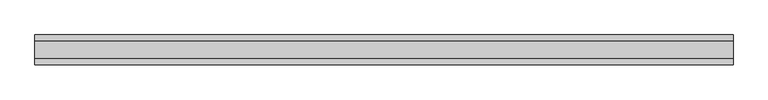
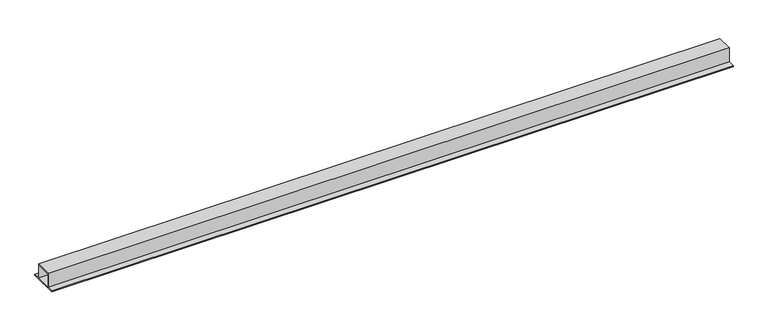
"""IFC4 building model written with IfcOpenShell, lengths in millimetres: beam geometry, NLRS_28_SF_LIB_stalen ligger THQ-AV-CWV-MMBS-SRP_gen_rsf : stalen ligger_gen__THQ_280x10-290x30-550x20."""

from ifc_helpers import new_model, si_unit, frame, origin, place, context, project, spatial, polyline, outline, extrude, source, transform, mapped, element, save


def beam_736acf17(model_context):
    return source(origin(), model_context, "Body", "SweptSolid", [
        extrude(outline(polyline([(143.5, 280.0), (143.5, 0.0), (263.5, 0.0), (263.5, -20.0), (-286.5, -20.0), (-286.5, 0.0), (-166.5, 0.0), (-166.5, 280.0), (143.5, 280.0)]), holes=[polyline([(133.5, 0.0), (133.5, 250.0), (-156.5, 250.0), (-156.5, 0.0), (133.5, 0.0)])]), frame((-6445.0, 0.0, 0.0), z_axis=(1.0, 0.0, 0.0), x_axis=(0.0, 1.0, 0.0)), (0.0, 0.0, 1.0), 12890.0),
    ])


if __name__ == "__main__":
    model = new_model("IFC4")
    model_context = context("Model", 3, world=origin())
    ifc_project = project(units=[si_unit("LENGTHUNIT", "METRE", prefix="MILLI")], contexts=[model_context])
    site = spatial("IfcSite", under=ifc_project)
    building = spatial("IfcBuilding", under=site)
    placement = place(None, origin())
    beam_shape = beam_736acf17(model_context)
    element("IfcBeam", 1, ObjectType="NLRS_28_SF_LIB_stalen ligger THQ-AV-CWV-MMBS-SRP_gen_rsf : stalen ligger_gen__THQ_280x10-290x30-550x20", at=placement, inside=building, context=model_context, shape_type="MappedRepresentation", body=[
        mapped(beam_shape, transform((0.0, 0.0, 0.0), x_axis=(1.0, 0.0, 0.0), y_axis=(0.0, 1.0, 0.0), z_axis=(0.0, 0.0, 1.0))),
    ])
    save(model, "model.ifc")

# Revit data of these elements
# Type "NLRS_28_SF_LIB_stalen ligger THQ-AV-CWV-MMBS-SRP_gen_rsf : stalen ligger_gen__THQ_280x10-290x30-550x20"
#   Type IfcGUID = "2GRbcre991teoKeCLB8MAm"
#   IfcExportAs = "IfcBeamType"
#   Type Comments = "THQ 280x10-290x30-550x20"
#   Model = " "
#   Manufacturer = " "
#   Fire Rating = " "
#   Description = "stalen ligger THQ 280x10-290x30-550x20"
#   Assembly Code = "28.11"
#   tw = 10 mm
#   tu = 20 mm
#   to = 30 mm
#   h = 280 mm
#   bu = 550 mm
#   bo = 290 mm
#   NLRS_C_lengte [instance default] = 1500 mm
#   Length [instance default] = 1500 mm
#   RSF_C_vullen_met_beton [instance default] = no
#   RSF_C_petligger = no
#   RSF_C_hoedligger = yes
#   Structural Material = NLRS_h2_staal_gen_rsf
#   Keynote = ""
# Element 1 (IfcBeam, "NLRS_28_SF_LIB_stalen ligger THQ-AV-CWV-MMBS-SRP_gen_rsf : stalen ligger_gen__THQ_280x10-290x30-550x20")
#   NLRS_C_lengte = 12890 mm
#   Materials on its faces: "NLRS_h2_staal_gen_rsf"
# Materials
#   "NLRS_h2_staal_gen_rsf": class "H - Metaal", colour RGB 189 187 185, transparency 0, Keynote = "h2", Manufacturer = "Revit Standards Foundation", URL = "www.revitstandards.org", Description = "staal", Cost = 0
